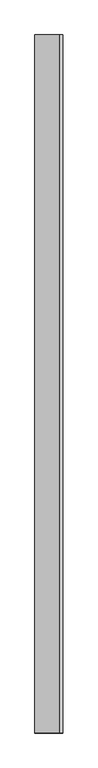
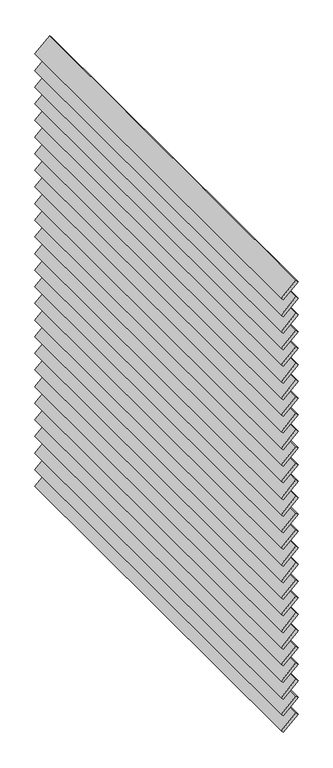
"""IFC4 building model written with IfcOpenShell, lengths in millimetres: proxy geometry, Door louver 1:Door louver 16505:300916 : Door louver 1:Door louver 16505:300916."""

from ifc_helpers import new_model, si_unit, frame, origin, place, context, project, spatial, polyline, outline, extrude, source, transform, mapped, element, save


def generic_models_1a776f2c(model_context):
    return source(origin(), model_context, "Body", "SweptSolid", [
        extrude(outline(polyline([(0.0, -88.6), (0.0, 0.0), (1847.6, 0.0), (1847.6, -88.6), (0.0, -88.6)])), frame((-3534.8574716, 6838.7838655, 34836.0547367), z_axis=(-0.692509227813749, 0.0, 0.7214090167116053), x_axis=(0.0, -1.0, 0.0)), (0.0, 0.0, 1.0), 13.8216714),
        extrude(outline(polyline([(0.0, -88.6), (0.0, 0.0), (1847.6, 0.0), (1847.6, -88.6), (0.0, -88.6)])), frame((-3534.8574716, 6838.7838655, 34759.8547367), z_axis=(-0.692509227813749, 0.0, 0.7214090167116053), x_axis=(0.0, -1.0, 0.0)), (0.0, 0.0, 1.0), 13.8216714),
        extrude(outline(polyline([(0.0, -88.6), (0.0, 0.0), (1847.6, 0.0), (1847.6, -88.6), (0.0, -88.6)])), frame((-3534.8574716, 6838.7838655, 34683.6547367), z_axis=(-0.692509227813749, 0.0, 0.7214090167116053), x_axis=(0.0, -1.0, 0.0)), (0.0, 0.0, 1.0), 13.8216714),
        extrude(outline(polyline([(0.0, -88.6), (0.0, 0.0), (1847.6, 0.0), (1847.6, -88.6), (0.0, -88.6)])), frame((-3534.8574716, 6838.7838655, 34607.4547367), z_axis=(-0.692509227813749, 0.0, 0.7214090167116053), x_axis=(0.0, -1.0, 0.0)), (0.0, 0.0, 1.0), 13.8216714),
        extrude(outline(polyline([(0.0, -88.6), (0.0, 0.0), (1847.6, 0.0), (1847.6, -88.6), (0.0, -88.6)])), frame((-3534.8574716, 6838.7838655, 34531.2547367), z_axis=(-0.692509227813749, 0.0, 0.7214090167116053), x_axis=(0.0, -1.0, 0.0)), (0.0, 0.0, 1.0), 13.8216714),
        extrude(outline(polyline([(0.0, -88.6), (0.0, 0.0), (1847.6, 0.0), (1847.6, -88.6), (0.0, -88.6)])), frame((-3534.8574716, 6838.7838655, 34455.0547367), z_axis=(-0.692509227813749, 0.0, 0.7214090167116053), x_axis=(0.0, -1.0, 0.0)), (0.0, 0.0, 1.0), 13.8216714),
        extrude(outline(polyline([(0.0, -88.6), (0.0, 0.0), (1847.6, 0.0), (1847.6, -88.6), (0.0, -88.6)])), frame((-3534.8574716, 6838.7838655, 34378.8547367), z_axis=(-0.692509227813749, 0.0, 0.7214090167116053), x_axis=(0.0, -1.0, 0.0)), (0.0, 0.0, 1.0), 13.8216714),
        extrude(outline(polyline([(0.0, -88.6), (0.0, 0.0), (1847.6, 0.0), (1847.6, -88.6), (0.0, -88.6)])), frame((-3534.8574716, 6838.7838655, 34302.6547367), z_axis=(-0.692509227813749, 0.0, 0.7214090167116053), x_axis=(0.0, -1.0, 0.0)), (0.0, 0.0, 1.0), 13.8216714),
        extrude(outline(polyline([(0.0, -88.6), (0.0, 0.0), (1847.6, 0.0), (1847.6, -88.6), (0.0, -88.6)])), frame((-3534.8574716, 6838.7838655, 34226.4547367), z_axis=(-0.692509227813749, 0.0, 0.7214090167116053), x_axis=(0.0, -1.0, 0.0)), (0.0, 0.0, 1.0), 13.8216714),
        extrude(outline(polyline([(0.0, -88.6), (0.0, 0.0), (1847.6, 0.0), (1847.6, -88.6), (0.0, -88.6)])), frame((-3534.8574716, 6838.7838655, 34150.2547367), z_axis=(-0.692509227813749, 0.0, 0.7214090167116053), x_axis=(0.0, -1.0, 0.0)), (0.0, 0.0, 1.0), 13.8216714),
        extrude(outline(polyline([(0.0, -88.6), (0.0, 0.0), (1847.6, 0.0), (1847.6, -88.6), (0.0, -88.6)])), frame((-3534.8574716, 6838.7838655, 34074.0547367), z_axis=(-0.692509227813749, 0.0, 0.7214090167116053), x_axis=(0.0, -1.0, 0.0)), (0.0, 0.0, 1.0), 13.8216714),
        extrude(outline(polyline([(0.0, -88.6), (0.0, 0.0), (1847.6, 0.0), (1847.6, -88.6), (0.0, -88.6)])), frame((-3534.8574716, 6838.7838655, 33997.8547367), z_axis=(-0.692509227813749, 0.0, 0.7214090167116053), x_axis=(0.0, -1.0, 0.0)), (0.0, 0.0, 1.0), 13.8216714),
        extrude(outline(polyline([(0.0, -88.6), (0.0, 0.0), (1847.6, 0.0), (1847.6, -88.6), (0.0, -88.6)])), frame((-3534.8574716, 6838.7838655, 33921.6547367), z_axis=(-0.692509227813749, 0.0, 0.7214090167116053), x_axis=(0.0, -1.0, 0.0)), (0.0, 0.0, 1.0), 13.8216714),
        extrude(outline(polyline([(0.0, -88.6), (0.0, 0.0), (1847.6, 0.0), (1847.6, -88.6), (0.0, -88.6)])), frame((-3534.8574716, 6838.7838655, 33845.4547367), z_axis=(-0.692509227813749, 0.0, 0.7214090167116053), x_axis=(0.0, -1.0, 0.0)), (0.0, 0.0, 1.0), 13.8216714),
        extrude(outline(polyline([(0.0, -88.6), (0.0, 0.0), (1847.6, 0.0), (1847.6, -88.6), (0.0, -88.6)])), frame((-3534.8574716, 6838.7838655, 33769.2547367), z_axis=(-0.692509227813749, 0.0, 0.7214090167116053), x_axis=(0.0, -1.0, 0.0)), (0.0, 0.0, 1.0), 13.8216714),
        extrude(outline(polyline([(0.0, -88.6), (0.0, 0.0), (1847.6, 0.0), (1847.6, -88.6), (0.0, -88.6)])), frame((-3534.8574716, 6838.7838655, 33693.0547367), z_axis=(-0.692509227813749, 0.0, 0.7214090167116053), x_axis=(0.0, -1.0, 0.0)), (0.0, 0.0, 1.0), 13.8216714),
        extrude(outline(polyline([(0.0, -88.6), (0.0, 0.0), (1847.6, 0.0), (1847.6, -88.6), (0.0, -88.6)])), frame((-3534.8574716, 6838.7838655, 33616.8547367), z_axis=(-0.692509227813749, 0.0, 0.7214090167116053), x_axis=(0.0, -1.0, 0.0)), (0.0, 0.0, 1.0), 13.8216714),
        extrude(outline(polyline([(0.0, -88.6), (0.0, 0.0), (1847.6, 0.0), (1847.6, -88.6), (0.0, -88.6)])), frame((-3534.8574716, 6838.7838655, 33540.6547367), z_axis=(-0.692509227813749, 0.0, 0.7214090167116053), x_axis=(0.0, -1.0, 0.0)), (0.0, 0.0, 1.0), 13.8216714),
        extrude(outline(polyline([(0.0, -88.6), (0.0, 0.0), (1847.6, 0.0), (1847.6, -88.6), (0.0, -88.6)])), frame((-3534.8574716, 6838.7838655, 33464.4547367), z_axis=(-0.692509227813749, 0.0, 0.7214090167116053), x_axis=(0.0, -1.0, 0.0)), (0.0, 0.0, 1.0), 13.8216714),
        extrude(outline(polyline([(0.0, -88.6), (0.0, 0.0), (1847.6, 0.0), (1847.6, -88.6), (0.0, -88.6)])), frame((-3534.8574716, 6838.7838655, 33388.2547367), z_axis=(-0.692509227813749, 0.0, 0.7214090167116053), x_axis=(0.0, -1.0, 0.0)), (0.0, 0.0, 1.0), 13.8216714),
        extrude(outline(polyline([(0.0, -88.6), (0.0, 0.0), (1847.6, 0.0), (1847.6, -88.6), (0.0, -88.6)])), frame((-3534.8574716, 6838.7838655, 33312.0547367), z_axis=(-0.692509227813749, 0.0, 0.7214090167116053), x_axis=(0.0, -1.0, 0.0)), (0.0, 0.0, 1.0), 13.8216714),
        extrude(outline(polyline([(0.0, -88.6), (0.0, 0.0), (1847.6, 0.0), (1847.6, -88.6), (0.0, -88.6)])), frame((-3534.8574716, 6838.7838655, 33235.8547367), z_axis=(-0.692509227813749, 0.0, 0.7214090167116053), x_axis=(0.0, -1.0, 0.0)), (0.0, 0.0, 1.0), 13.8216714),
        extrude(outline(polyline([(0.0, -88.6), (0.0, 0.0), (1847.6, 0.0), (1847.6, -88.6), (0.0, -88.6)])), frame((-3534.8574716, 6838.7838655, 33159.6547367), z_axis=(-0.692509227813749, 0.0, 0.7214090167116053), x_axis=(0.0, -1.0, 0.0)), (0.0, 0.0, 1.0), 13.8216714),
        extrude(outline(polyline([(0.0, -88.6), (0.0, 0.0), (1847.6, 0.0), (1847.6, -88.6), (0.0, -88.6)])), frame((-3534.8574716, 6838.7838655, 33083.4547367), z_axis=(-0.692509227813749, 0.0, 0.7214090167116053), x_axis=(0.0, -1.0, 0.0)), (0.0, 0.0, 1.0), 13.8216714),
        extrude(outline(polyline([(0.0, -88.6), (0.0, 0.0), (1847.6, 0.0), (1847.6, -88.6), (0.0, -88.6)])), frame((-3534.8574716, 6838.7838655, 33007.2547367), z_axis=(-0.692509227813749, 0.0, 0.7214090167116053), x_axis=(0.0, -1.0, 0.0)), (0.0, 0.0, 1.0), 13.8216714),
        extrude(outline(polyline([(0.0, -88.6), (0.0, 0.0), (1847.6, 0.0), (1847.6, -88.6), (0.0, -88.6)])), frame((-3534.8574716, 6838.7838655, 32931.0547367), z_axis=(-0.692509227813749, 0.0, 0.7214090167116053), x_axis=(0.0, -1.0, 0.0)), (0.0, 0.0, 1.0), 13.8216714),
        extrude(outline(polyline([(0.0, -88.6), (0.0, 0.0), (1847.6, 0.0), (1847.6, -88.6), (0.0, -88.6)])), frame((-3534.8574716, 6838.7838655, 32854.8547367), z_axis=(-0.692509227813749, 0.0, 0.7214090167116053), x_axis=(0.0, -1.0, 0.0)), (0.0, 0.0, 1.0), 13.8216714),
    ])


if __name__ == "__main__":
    model = new_model("IFC4")
    model_context = context("Model", 3, world=origin())
    ifc_project = project(units=[si_unit("LENGTHUNIT", "METRE", prefix="MILLI")], contexts=[model_context])
    site = spatial("IfcSite", under=ifc_project)
    building = spatial("IfcBuilding", under=site)
    placement = place(None, origin())
    generic_models_shape = generic_models_1a776f2c(model_context)
    element("IfcBuildingElementProxy", 1, Name="Door louver 1:Door louver 16505:300916 : Door louver 1:Door louver 16505:300916", ObjectType="Door louver 1:Door louver 16505:300916 : Door louver 1:Door louver 16505:300916", at=placement, inside=building, context=model_context, shape_type="MappedRepresentation", body=[
        mapped(generic_models_shape, transform((0.0, 0.0, 0.0), x_axis=(1.0, 0.0, 0.0), y_axis=(0.0, 1.0, 0.0), z_axis=(0.0, 0.0, 1.0))),
    ])
    save(model, "model.ifc")

# Revit data of these elements
# Type "Door louver 1:Door louver 16505:300916 : Door louver 1:Door louver 16505:300916"
#   NameOverride = "Door louver 1:Door louver 16505:300916"
#   ObjectTypeOverride = "Door louver 1:Door louver 16505"
#   Reference = "Door louver 16505"
#   Category = "Generic Models"
#   Tag = "300916"
# Element 1 (IfcBuildingElementProxy, "Door louver 1:Door louver 16505:300916 : Door louver 1:Door louver 16505:300916")
#   Materials on its faces: "WOODEN LOUVERS (SPEC T. B. D.)"
# Materials
#   "WOODEN LOUVERS (SPEC T. B. D.)": class "Unassigned", colour RGB 148 103 60, transparency 0, Cost = 0
